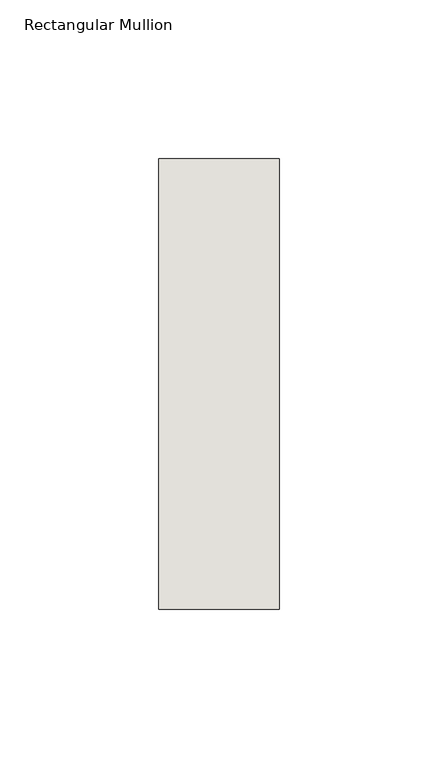
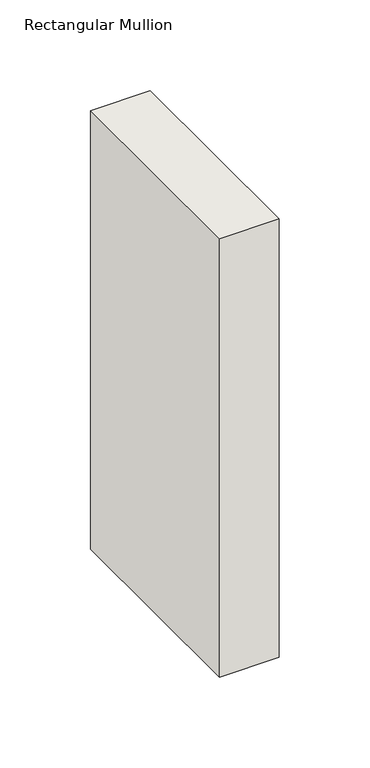
"""IFC4 building model written with IfcOpenShell, lengths in millimetres: wall geometry, Rectangular Mullion : NLRS_21_CWM_hsb-regel 38x142_gen_rsf."""

from ifc_helpers import new_model, si_unit, frame, origin, place, context, project, spatial, polyline, outline, extrude, source, transform, mapped, element, save


def rectangular_mullion_e102e68a(model_context):
    return source(origin(), model_context, "Body", "SweptSolid", [
        extrude(outline(polyline([(-38.0, -71.0), (-38.0, 71.0), (0.0, 71.0), (0.0, -71.0), (-38.0, -71.0)])), frame((0.0, 0.0, -295.0), z_axis=(0.0, 0.0, 1.0), x_axis=(1.0, 0.0, 0.0)), (0.0, 0.0, 1.0), 295.0),
    ])


if __name__ == "__main__":
    model = new_model("IFC4")
    model_context = context("Model", 3, world=origin())
    ifc_project = project(units=[si_unit("LENGTHUNIT", "METRE", prefix="MILLI")], contexts=[model_context])
    site = spatial("IfcSite", under=ifc_project)
    building = spatial("IfcBuilding", under=site)
    placement = place(None, origin())
    rectangular_mullion_shape = rectangular_mullion_e102e68a(model_context)
    element("IfcWall", 1, ObjectType="Rectangular Mullion : NLRS_21_CWM_hsb-regel 38x142_gen_rsf", at=placement, inside=building, context=model_context, shape_type="MappedRepresentation", body=[
        mapped(rectangular_mullion_shape, transform((0.0, 0.0, 0.0), x_axis=(1.0, 0.0, 0.0), y_axis=(0.0, 1.0, 0.0), z_axis=(0.0, 0.0, 1.0))),
    ])
    save(model, "model.ifc")

# Revit data of these elements
# Type "Rectangular Mullion : NLRS_21_CWM_hsb-regel 38x142_gen_rsf"
#   Type IfcGUID = "07M7mRoiH1CR8m_RSKIwpF"
#   Assembly Code = "21.10"
#   IfcExportAs = "IfcWall"
#   built-in parameter 1007322 = 0.465879 (stored number, unit not read)
#   built-in parameter 1007321 = 0.062336 (stored number, unit not read)
#   built-in parameter 1007320 = 0.062336 (stored number, unit not read)
# Element 1 (IfcWall, "Rectangular Mullion : NLRS_21_CWM_hsb-regel 38x142_gen_rsf")
#   Materials on its faces: "NLRS_i2_hout naaldhout vuren_gen_rsf"
# Materials
#   "NLRS_i2_hout naaldhout vuren_gen_rsf": class "I - Hout", colour RGB 234 199 147, transparency 0, Keynote = "i2", Manufacturer = "Revit Standards Foundation", URL = "www.revitstandards.org", Description = "hout vuren", Cost = 0
